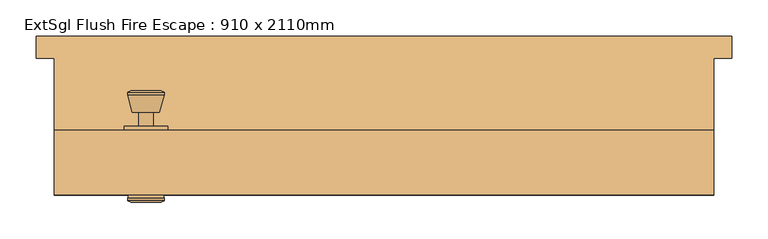
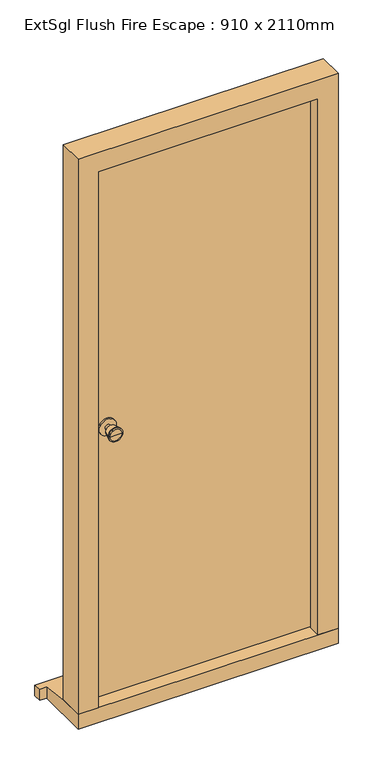
"""IFC4 building model written with IfcOpenShell, lengths in millimetres: door geometry, ExtSgl Flush Fire Escape : 910 x 2110mm."""

from ifc_helpers import new_model, si_unit, point, frame, frame_2d, origin, place, context, project, spatial, polyline, circle_curve, trimmed, segment, composite_curve, outline, extrude, faceted_brep, source, transform, mapped, element, save
from ifc_brep_helpers import plane_surface, cylinder_surface, revolved_surface, advanced_brep


def extsgl_flush_fire_escape_910_x_2110mm_612fc41a(model_context):
    return source(origin(), model_context, "Body", "SolidModel", [
        advanced_brep(
        [(-328.5, 121.0, 1050.0), (-338.5, 121.0, 1050.0), (-318.5, 121.0, 1050.0), (-308.0241324, 170.0, 1050.0), (-348.9758676, 170.0, 1050.0), (-328.5, 170.0, 1050.0), (-303.5, 168.1721319, 1050.0), (-353.5, 168.1721319, 1050.0), (-303.5, 164.7084537, 1050.0), (-353.5, 164.7084537, 1050.0), (-309.863764, 140.0, 1050.0), (-347.136236, 140.0, 1050.0), (-318.5, 140.0, 1050.0), (-338.5, 140.0, 1050.0)],
        [
            (0, 1),
            (1, 2, circle_curve(frame((-328.5, 121.0, 1050.0), z_axis=(0.0, -1.0, 0.0), x_axis=(-1.0, 0.0, 0.0)), 10.0)),
            (2, 0),
            (2, 1, circle_curve(frame((-328.5, 121.0, 1050.0), z_axis=(0.0, -1.0, 0.0), x_axis=(-1.0, 0.0, 0.0)), 10.0)),
            (3, 4, circle_curve(frame((-328.5, 170.0, 1050.0), z_axis=(0.0, 1.0, 0.0), x_axis=(-1.0, 0.0, 0.0)), 20.4758676)),
            (4, 5),
            (5, 3),
            (4, 3, circle_curve(frame((-328.5, 170.0, 1050.0), z_axis=(0.0, 1.0, 0.0), x_axis=(-1.0, 0.0, 0.0)), 20.4758676)),
            (6, 7, circle_curve(frame((-328.5, 168.1721319, 1050.0), z_axis=(0.0, 1.0, 0.0), x_axis=(-1.0, 0.0, 0.0)), 25.0)),
            (7, 4),
            (3, 6),
            (7, 6, circle_curve(frame((-328.5, 168.1721319, 1050.0), z_axis=(0.0, 1.0, 0.0), x_axis=(-1.0, 0.0, 0.0)), 25.0)),
            (8, 9, circle_curve(frame((-328.5, 164.7084537, 1050.0), z_axis=(0.0, 1.0, 0.0), x_axis=(-1.0, 0.0, 0.0)), 25.0)),
            (9, 7),
            (6, 8),
            (9, 8, circle_curve(frame((-328.5, 164.7084537, 1050.0), z_axis=(0.0, 1.0, 0.0), x_axis=(-1.0, 0.0, 0.0)), 25.0)),
            (10, 11, circle_curve(frame((-328.5, 140.0, 1050.0), z_axis=(0.0, 1.0, 0.0), x_axis=(-1.0, 0.0, 0.0)), 18.636236)),
            (11, 9),
            (8, 10),
            (11, 10, circle_curve(frame((-328.5, 140.0, 1050.0), z_axis=(0.0, 1.0, 0.0), x_axis=(-1.0, 0.0, 0.0)), 18.636236)),
            (12, 13, circle_curve(frame((-328.5, 140.0, 1050.0), z_axis=(0.0, 1.0, 0.0), x_axis=(-1.0, 0.0, 0.0)), 10.0)),
            (13, 11),
            (10, 12),
            (13, 12, circle_curve(frame((-328.5, 140.0, 1050.0), z_axis=(0.0, 1.0, 0.0), x_axis=(-1.0, 0.0, 0.0)), 10.0)),
            (1, 13),
            (12, 2),
        ],
        [
            plane_surface(frame((-328.5, 121.0, 1050.0), z_axis=(0.0, -1.0, 0.0), x_axis=(-1.0, 0.0, 0.0))),
            plane_surface(frame((-328.5, 170.0, 1050.0), z_axis=(0.0, 1.0, 0.0), x_axis=(-1.0, 0.0, 0.0))),
            revolved_surface(polyline([(-348.9758676, 170.0, 1050.0), (-353.5, 168.1721319, 1050.0)]), (-328.5, 121.0, 1050.0), (0.0, -1.0, 0.0)),
            cylinder_surface(frame((-328.5, 121.0, 1050.0), z_axis=(0.0, -1.0, 0.0), x_axis=(-1.0, 0.0, 0.0)), 25.0),
            revolved_surface(polyline([(-353.5, 164.7084537, 1050.0), (-347.136236, 140.0, 1050.0)]), (-328.5, 121.0, 1050.0), (0.0, -1.0, 0.0)),
            plane_surface(frame((-328.5, 140.0, 1050.0), z_axis=(0.0, -1.0, 0.0), x_axis=(-1.0, 0.0, 0.0))),
            cylinder_surface(frame((-328.5, 121.0, 1050.0), z_axis=(0.0, -1.0, 0.0), x_axis=(-1.0, 0.0, 0.0)), 10.0),
        ],
        [
            (0, [[1, 2, 3]]),
            (0, [[-3, 4, -1]]),
            (1, [[5, 6, 7]]),
            (1, [[8, -7, -6]]),
            (2, [[9, 10, -5, 11]]),
            (2, [[12, -11, -8, -10]]),
            (3, [[13, 14, -9, 15]]),
            (3, [[16, -15, -12, -14]]),
            (4, [[17, 18, -13, 19]]),
            (4, [[20, -19, -16, -18]]),
            (5, [[21, 22, -17, 23]]),
            (5, [[24, -23, -20, -22]]),
            (6, [[-2, 25, -21, 26]]),
            (6, [[-4, -26, -24, -25]]),
        ],
    ),
        extrude(outline(composite_curve([segment(trimmed(circle_curve(frame_2d((1050.0, -328.5)), 30.0), [point((1050.0, -358.5))], [point((1050.0, -298.5))], False, "CARTESIAN"), True, "CONTINUOUS"), segment(trimmed(circle_curve(frame_2d((1050.0, -328.5)), 30.0), [point((1050.0, -298.5))], [point((1050.0, -358.5))], False, "CARTESIAN"), True, "CONTINUOUS")], self_intersect=False)), frame((0.0, 115.0, 0.0), z_axis=(0.0, 1.0, 0.0), x_axis=(0.0, 0.0, 1.0)), (0.0, 0.0, 1.0), 6.0),
        advanced_brep(
        [(-328.5, 65.0, 1050.0), (-318.5, 65.0, 1050.0), (-338.5, 65.0, 1050.0), (-308.0241324, 16.0, 1050.0), (-328.5, 16.0, 1050.0), (-348.9758676, 16.0, 1050.0), (-303.5, 17.8278681, 1050.0), (-353.5, 17.8278681, 1050.0), (-303.5, 21.2915463, 1050.0), (-353.5, 21.2915463, 1050.0), (-309.863764, 46.0, 1050.0), (-347.136236, 46.0, 1050.0), (-318.5, 46.0, 1050.0), (-338.5, 46.0, 1050.0)],
        [
            (0, 1),
            (1, 2, circle_curve(frame((-328.5, 65.0, 1050.0), z_axis=(0.0, 1.0, 0.0), x_axis=(-1.0, 0.0, 0.0)), 10.0)),
            (2, 0),
            (2, 1, circle_curve(frame((-328.5, 65.0, 1050.0), z_axis=(0.0, 1.0, 0.0), x_axis=(-1.0, 0.0, 0.0)), 10.0)),
            (3, 4),
            (4, 5),
            (5, 3, circle_curve(frame((-328.5, 16.0, 1050.0), z_axis=(0.0, -1.0, 0.0), x_axis=(-1.0, 0.0, 0.0)), 20.4758676)),
            (3, 5, circle_curve(frame((-328.5, 16.0, 1050.0), z_axis=(0.0, -1.0, 0.0), x_axis=(-1.0, 0.0, 0.0)), 20.4758676)),
            (6, 3),
            (5, 7),
            (7, 6, circle_curve(frame((-328.5, 17.8278681, 1050.0), z_axis=(0.0, -1.0, 0.0), x_axis=(-1.0, 0.0, 0.0)), 25.0)),
            (6, 7, circle_curve(frame((-328.5, 17.8278681, 1050.0), z_axis=(0.0, -1.0, 0.0), x_axis=(-1.0, 0.0, 0.0)), 25.0)),
            (8, 6),
            (7, 9),
            (9, 8, circle_curve(frame((-328.5, 21.2915463, 1050.0), z_axis=(0.0, -1.0, 0.0), x_axis=(-1.0, 0.0, 0.0)), 25.0)),
            (8, 9, circle_curve(frame((-328.5, 21.2915463, 1050.0), z_axis=(0.0, -1.0, 0.0), x_axis=(-1.0, 0.0, 0.0)), 25.0)),
            (10, 8),
            (9, 11),
            (11, 10, circle_curve(frame((-328.5, 46.0, 1050.0), z_axis=(0.0, -1.0, 0.0), x_axis=(-1.0, 0.0, 0.0)), 18.636236)),
            (10, 11, circle_curve(frame((-328.5, 46.0, 1050.0), z_axis=(0.0, -1.0, 0.0), x_axis=(-1.0, 0.0, 0.0)), 18.636236)),
            (12, 10),
            (11, 13),
            (13, 12, circle_curve(frame((-328.5, 46.0, 1050.0), z_axis=(0.0, -1.0, 0.0), x_axis=(-1.0, 0.0, 0.0)), 10.0)),
            (12, 13, circle_curve(frame((-328.5, 46.0, 1050.0), z_axis=(0.0, -1.0, 0.0), x_axis=(-1.0, 0.0, 0.0)), 10.0)),
            (1, 12),
            (13, 2),
        ],
        [
            plane_surface(frame((-328.5, 65.0, 1050.0), z_axis=(0.0, 1.0, 0.0), x_axis=(-1.0, 0.0, 0.0))),
            plane_surface(frame((-328.5, 16.0, 1050.0), z_axis=(0.0, -1.0, 0.0), x_axis=(-1.0, 0.0, 0.0))),
            revolved_surface(polyline([(-348.9758676, 16.0, 1050.0), (-353.5, 17.8278681, 1050.0)]), (-328.5, 65.0, 1050.0), (0.0, 1.0, 0.0)),
            cylinder_surface(frame((-328.5, 65.0, 1050.0), z_axis=(0.0, 1.0, 0.0), x_axis=(-1.0, 0.0, 0.0)), 25.0),
            revolved_surface(polyline([(-353.5, 21.2915463, 1050.0), (-347.136236, 46.0, 1050.0)]), (-328.5, 65.0, 1050.0), (0.0, 1.0, 0.0)),
            plane_surface(frame((-328.5, 46.0, 1050.0), z_axis=(0.0, 1.0, 0.0), x_axis=(-1.0, 0.0, 0.0))),
            cylinder_surface(frame((-328.5, 65.0, 1050.0), z_axis=(0.0, 1.0, 0.0), x_axis=(-1.0, 0.0, 0.0)), 10.0),
        ],
        [
            (0, [[1, 2, 3]]),
            (0, [[-3, 4, -1]]),
            (1, [[5, 6, 7]]),
            (1, [[-6, -5, 8]]),
            (2, [[9, -7, 10, 11]]),
            (2, [[-10, -8, -9, 12]]),
            (3, [[13, -11, 14, 15]]),
            (3, [[-14, -12, -13, 16]]),
            (4, [[17, -15, 18, 19]]),
            (4, [[-18, -16, -17, 20]]),
            (5, [[21, -19, 22, 23]]),
            (5, [[-22, -20, -21, 24]]),
            (6, [[25, -23, 26, -2]]),
            (6, [[-26, -24, -25, -4]]),
        ],
    ),
        extrude(outline(composite_curve([segment(trimmed(circle_curve(frame_2d((1050.0, -328.5)), 30.0), [point((1050.0, -358.5))], [point((1050.0, -298.5))], False, "CARTESIAN"), True, "CONTINUOUS"), segment(trimmed(circle_curve(frame_2d((1050.0, -328.5)), 30.0), [point((1050.0, -298.5))], [point((1050.0, -358.5))], False, "CARTESIAN"), True, "CONTINUOUS")], self_intersect=False)), frame((0.0, 65.0, 0.0), z_axis=(0.0, 1.0, 0.0), x_axis=(0.0, 0.0, 1.0)), (0.0, 0.0, 1.0), 6.0),
        faceted_brep([(406.5, 115.0, 54.5), (455.0, 115.0, 54.5), (455.0, 26.0, 54.5), (384.5, 26.0, 54.5), (384.5, 68.0, 54.5), (406.5, 68.0, 54.5), (406.5, 115.0, 2061.5), (-406.5, 115.0, 2061.5), (-406.5, 115.0, 54.5), (-455.0, 115.0, 54.5), (-455.0, 115.0, 2110.0), (455.0, 115.0, 2110.0), (455.0, 26.0, 2110.0), (-455.0, 26.0, 2110.0), (-455.0, 26.0, 54.5), (-384.5, 26.0, 54.5), (-384.5, 26.0, 2039.5), (384.5, 26.0, 2039.5), (384.5, 68.0, 2039.5), (-384.5, 68.0, 2039.5), (-384.5, 68.0, 54.5), (-406.5, 68.0, 54.5), (-406.5, 68.0, 2061.5), (406.5, 68.0, 2061.5)], [[[0, 1, 2, 3, 4, 5]], [[1, 0, 6, 7, 8, 9, 10, 11]], [[2, 1, 11, 12]], [[3, 2, 12, 13, 14, 15, 16, 17]], [[4, 3, 17, 18]], [[5, 4, 18, 19, 20, 21, 22, 23]], [[0, 5, 23, 6]], [[7, 22, 21, 8]], [[8, 21, 20, 15, 14, 9]], [[13, 10, 9, 14]], [[19, 16, 15, 20]], [[12, 11, 10, 13]], [[18, 17, 16, 19]], [[6, 23, 22, 7]]]),
        faceted_brep([(480.0, 245.0, 0.0), (480.0, 245.0, 38.5947221), (480.0, 215.0, 42.2651709), (480.0, 215.0, 0.0), (-480.0, 245.0, 38.5947221), (-480.0, 245.0, 0.0), (-480.0, 215.0, 0.0), (-480.0, 215.0, 42.2651709), (455.0, 215.0, 0.0), (455.0, 26.0, 0.0), (-455.0, 26.0, 0.0), (-455.0, 215.0, 0.0), (-455.0, 215.0, 42.2651709), (-455.0, 115.0, 54.5), (455.0, 115.0, 54.5), (455.0, 215.0, 42.2651709), (-455.0, 26.0, 54.5), (455.0, 26.0, 54.5)], [[[0, 1, 2, 3]], [[4, 5, 6, 7]], [[5, 0, 3, 8, 9, 10, 11, 6]], [[1, 0, 5, 4]], [[1, 4, 7, 12, 13, 14, 15, 2]], [[13, 16, 17, 14]], [[16, 10, 9, 17]], [[12, 11, 10, 16, 13]], [[11, 12, 7, 6]], [[8, 15, 14, 17, 9]], [[15, 8, 3, 2]]]),
        extrude(outline(polyline([(403.5, 71.0), (-404.4250294, 71.0), (-404.4250294, 115.0), (403.5, 115.0), (403.5, 71.0)])), frame((0.0, 0.0, 58.5), z_axis=(0.0, 0.0, 1.0), x_axis=(1.0, 0.0, 0.0)), (0.0, 0.0, 1.0), 2000.0),
    ])


if __name__ == "__main__":
    model = new_model("IFC4")
    model_context = context("Model", 3, world=origin())
    ifc_project = project(units=[si_unit("LENGTHUNIT", "METRE", prefix="MILLI")], contexts=[model_context])
    site = spatial("IfcSite", under=ifc_project)
    building = spatial("IfcBuilding", under=site)
    placement = place(None, origin())
    extsgl_flush_fire_escape_910_x_2110mm_shape = extsgl_flush_fire_escape_910_x_2110mm_612fc41a(model_context)
    element("IfcDoor", 1, ObjectType="ExtSgl Flush Fire Escape : 910 x 2110mm", at=placement, inside=building, context=model_context, shape_type="MappedRepresentation", body=[
        mapped(extsgl_flush_fire_escape_910_x_2110mm_shape, transform((0.0, 0.0, 0.0), x_axis=(1.0, 0.0, 0.0), y_axis=(0.0, 1.0, 0.0), z_axis=(0.0, 0.0, 1.0))),
    ])
    save(model, "model.ifc")

# Revit data of these elements
# Type "ExtSgl Flush Fire Escape : 910 x 2110mm"
#   Description = "Fire Escape Door"
#   Type Mark = "57"
#   Type Comments = "External Single"
#   Operation = "SingleSwingRight"
#   Construction Type Id = "MDOOR"
#   Keynote = "L20"
#   Analytic Construction = "Metal"
#   Wrap Layers (Int) from Ext = 177.5 mm
#   Wrap Layers (Ext) from Ext = 102.5 mm
#   Thickness = 44 mm
#   Rough Width = 910 mm
#   Rough Height = 2110 mm
#   O/A Frame Width = 64 mm
#   Heat Transfer Coefficient (U) = 3.7021 W/(m²·K)
#   Handle Z Distance = 1050 mm
#   FrameWidth = 42 mm
#   FrameOffset - External = 100 mm
#   FrameDepth = 89 mm
#   Door Panel Width = 807 mm
#   Door Panel Thickness = 44 mm
#   Door Panel Height = 2000 mm
#   Cill Thickness = 54.5 mm
#   Cill Projection = 30 mm
#   Handle X Distance = 75 mm
#   Height = 2110 mm
#   Structural Tolerance = 6.5 mm
#   Tolerance = 3 mm
#   Undercut = 4 mm
#   Width = 910 mm
#   Cill Extension = 25 mm
#   Cavity Closer Width = 75 mm
#   Cavity Closer Offset from Ext = 120 mm
#   Cavity Closer Depth = 95 mm
#   Vis - Ironmongery = yes
#   Vis - Cavity Closers = yes
#   Define Thermal Properties by = 1
#   Function = 1
#   Material Door = Door - Panel
#   Material Frame = Door - Frame/Mullion
#   Material Ironmongery = Door - Handle
#   Visual Light Transmittance = 0
#   Solar Heat Gain Coefficient = 0
#   Wall Closure = (empty or 0)
# Element 1 (IfcDoor, "ExtSgl Flush Fire Escape : 910 x 2110mm")
#   Materials on its faces: "Door - Handle", "Door - Frame/Mullion", "Door - Panel"
# Materials
#   "Door - Panel": class "Wood", colour RGB 210 159 95, transparency 0, Keynote = "L20"
#   "Door - Frame/Mullion": class "Wood", colour RGB 212 179 113, transparency 0, Keynote = "L20"
#   "Door - Handle": class "Miscellaneous", colour RGB 0 0 0, transparency 0, Keynote = "P21"
